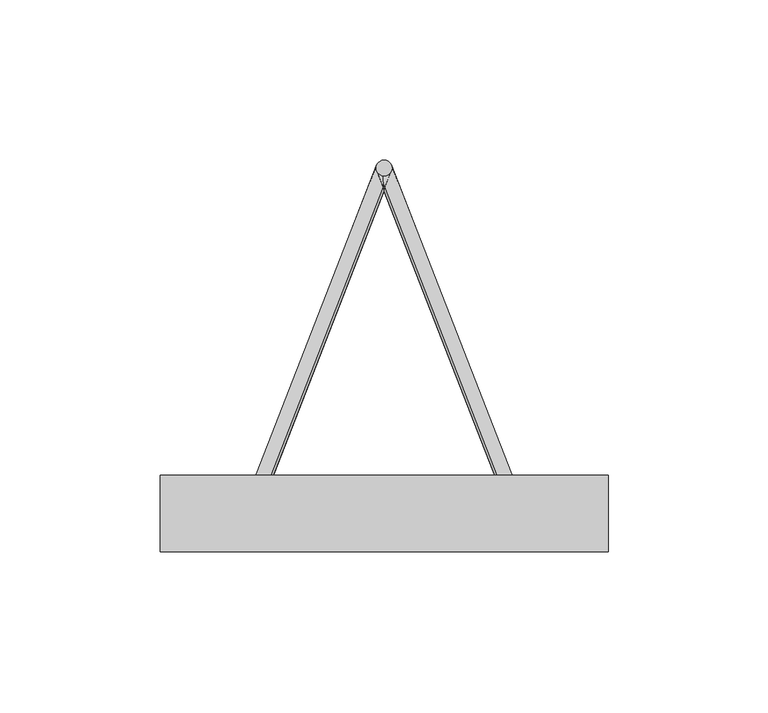
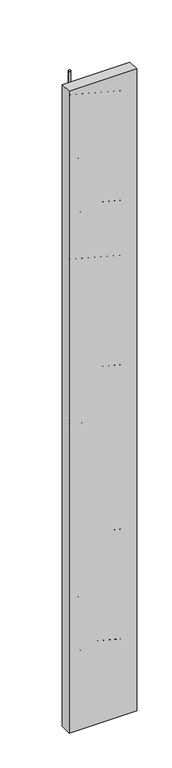
"""IFC4 building model written with IfcOpenShell, lengths in millimetres: proxy geometry, Vigota 1 (Pano 21) (Mf = 156)."""

from ifc_helpers import new_model, si_unit, point, frame, frame_2d, origin, origin_with_axes, origin_2d, place, context, project, spatial, polyline, circle_curve, trimmed, segment, composite_curve, outline, extrude, source, transform, mapped, element, save


def structural_framing_4ac9c4cf(model_context):
    return source(origin(), model_context, "Body", "SweptSolid", [
        extrude(outline(polyline([(-70.0, 12.0), (70.0, 12.0), (70.0, -12.0), (-70.0, -12.0), (-70.0, 12.0)])), origin_with_axes(), (0.0, 0.0, 1.0), 1404.99893),
        extrude(outline(composite_curve([segment(trimmed(circle_curve(frame_2d((42.0, 0.0)), 2.5), [point((44.5, 0.0))], [point((39.5, 0.0))], False, "CARTESIAN"), True, "CONTINUOUS"), segment(trimmed(circle_curve(frame_2d((42.0, 0.0)), 2.5), [point((39.5, 0.0))], [point((44.5, 0.0))], False, "CARTESIAN"), True, "CONTINUOUS")], self_intersect=False)), frame((0.0, 0.0, 28.0), z_axis=(0.0, 0.0, 1.0), x_axis=(1.0, 0.0, 0.0)), (0.0, 0.0, 1.0), 1348.99893),
        extrude(outline(composite_curve([segment(trimmed(circle_curve(frame_2d((0.0, 108.0)), 2.5), [point((2.5, 108.0))], [point((-2.5, 108.0))], False, "CARTESIAN"), True, "CONTINUOUS"), segment(trimmed(circle_curve(frame_2d((0.0, 108.0)), 2.5), [point((-2.5, 108.0))], [point((2.5, 108.0))], False, "CARTESIAN"), True, "CONTINUOUS")], self_intersect=False)), frame((0.0, 0.0, 52.499465), z_axis=(0.0, 0.0, 1.0), x_axis=(1.0, 0.0, 0.0)), (0.0, 0.0, 1.0), 1300.0),
        extrude(outline(composite_curve([segment(trimmed(circle_curve(origin_2d(), 2.5), [point((2.5, 0.0))], [point((-2.5, 0.0))], False, "CARTESIAN"), True, "CONTINUOUS"), segment(trimmed(circle_curve(origin_2d(), 2.5), [point((-2.5, 0.0))], [point((2.5, 0.0))], False, "CARTESIAN"), True, "CONTINUOUS")], self_intersect=False)), frame((42.0, 0.0, 42.499465), z_axis=(-0.3218603428886276, 0.8276408817707567, 0.4598004898837537), x_axis=(0.8192319205108605, -3.936835275445103e-11, 0.5734623443750141)), (0.0, 0.0, 1.0), 130.491379),
        extrude(outline(composite_curve([segment(trimmed(circle_curve(origin_2d(), 2.5), [point((2.5, 0.0))], [point((-2.5, 0.0))], False, "CARTESIAN"), True, "CONTINUOUS"), segment(trimmed(circle_curve(origin_2d(), 2.5), [point((-2.5, 0.0))], [point((2.5, 0.0))], False, "CARTESIAN"), True, "CONTINUOUS")], self_intersect=False)), frame((0.0, 108.0, 102.499465), z_axis=(0.3218603428886276, -0.8276408817707567, 0.4598004898837537), x_axis=(0.8192319205108605, -3.936835275445103e-11, -0.5734623443750141)), (0.0, 0.0, 1.0), 130.491379),
        extrude(outline(composite_curve([segment(trimmed(circle_curve(origin_2d(), 2.5), [point((2.5, 0.0))], [point((-2.5, 0.0))], False, "CARTESIAN"), True, "CONTINUOUS"), segment(trimmed(circle_curve(origin_2d(), 2.5), [point((-2.5, 0.0))], [point((2.5, 0.0))], False, "CARTESIAN"), True, "CONTINUOUS")], self_intersect=False)), frame((42.0, 0.0, 162.499465), z_axis=(-0.3218603428886276, 0.8276408817707567, 0.4598004898837537), x_axis=(0.8192319205108605, -3.936835275445103e-11, 0.5734623443750141)), (0.0, 0.0, 1.0), 130.491379),
        extrude(outline(composite_curve([segment(trimmed(circle_curve(origin_2d(), 2.5), [point((2.5, 0.0))], [point((-2.5, 0.0))], False, "CARTESIAN"), True, "CONTINUOUS"), segment(trimmed(circle_curve(origin_2d(), 2.5), [point((-2.5, 0.0))], [point((2.5, 0.0))], False, "CARTESIAN"), True, "CONTINUOUS")], self_intersect=False)), frame((0.0, 108.0, 222.499465), z_axis=(0.3218603428886276, -0.8276408817707567, 0.4598004898837537), x_axis=(0.8192319205108605, -3.936835275445103e-11, -0.5734623443750141)), (0.0, 0.0, 1.0), 130.491379),
        extrude(outline(composite_curve([segment(trimmed(circle_curve(origin_2d(), 2.5), [point((2.5, 0.0))], [point((-2.5, 0.0))], False, "CARTESIAN"), True, "CONTINUOUS"), segment(trimmed(circle_curve(origin_2d(), 2.5), [point((-2.5, 0.0))], [point((2.5, 0.0))], False, "CARTESIAN"), True, "CONTINUOUS")], self_intersect=False)), frame((42.0, 0.0, 282.499465), z_axis=(-0.3218603428886276, 0.8276408817707567, 0.4598004898837537), x_axis=(0.8192319205108605, -3.936835275445103e-11, 0.5734623443750141)), (0.0, 0.0, 1.0), 130.491379),
        extrude(outline(composite_curve([segment(trimmed(circle_curve(origin_2d(), 2.5), [point((2.5, 0.0))], [point((-2.5, 0.0))], False, "CARTESIAN"), True, "CONTINUOUS"), segment(trimmed(circle_curve(origin_2d(), 2.5), [point((-2.5, 0.0))], [point((2.5, 0.0))], False, "CARTESIAN"), True, "CONTINUOUS")], self_intersect=False)), frame((0.0, 108.0, 342.499465), z_axis=(0.3218603428886276, -0.8276408817707567, 0.4598004898837537), x_axis=(0.8192319205108605, -3.936835275445103e-11, -0.5734623443750141)), (0.0, 0.0, 1.0), 130.491379),
        extrude(outline(composite_curve([segment(trimmed(circle_curve(origin_2d(), 2.5), [point((2.5, 0.0))], [point((-2.5, 0.0))], False, "CARTESIAN"), True, "CONTINUOUS"), segment(trimmed(circle_curve(origin_2d(), 2.5), [point((-2.5, 0.0))], [point((2.5, 0.0))], False, "CARTESIAN"), True, "CONTINUOUS")], self_intersect=False)), frame((42.0, 0.0, 402.499465), z_axis=(-0.3218603428886276, 0.8276408817707567, 0.4598004898837537), x_axis=(0.8192319205108605, -3.936835275445103e-11, 0.5734623443750141)), (0.0, 0.0, 1.0), 130.491379),
        extrude(outline(composite_curve([segment(trimmed(circle_curve(origin_2d(), 2.5), [point((2.5, 0.0))], [point((-2.5, 0.0))], False, "CARTESIAN"), True, "CONTINUOUS"), segment(trimmed(circle_curve(origin_2d(), 2.5), [point((-2.5, 0.0))], [point((2.5, 0.0))], False, "CARTESIAN"), True, "CONTINUOUS")], self_intersect=False)), frame((0.0, 108.0, 462.499465), z_axis=(0.3218603428886276, -0.8276408817707567, 0.4598004898837537), x_axis=(0.8192319205108605, -3.936835275445103e-11, -0.5734623443750141)), (0.0, 0.0, 1.0), 130.491379),
        extrude(outline(composite_curve([segment(trimmed(circle_curve(origin_2d(), 2.5), [point((2.5, 0.0))], [point((-2.5, 0.0))], False, "CARTESIAN"), True, "CONTINUOUS"), segment(trimmed(circle_curve(origin_2d(), 2.5), [point((-2.5, 0.0))], [point((2.5, 0.0))], False, "CARTESIAN"), True, "CONTINUOUS")], self_intersect=False)), frame((42.0, 0.0, 522.499465), z_axis=(-0.3218603428886276, 0.8276408817707567, 0.4598004898837537), x_axis=(0.8192319205108605, -3.936835275445103e-11, 0.5734623443750141)), (0.0, 0.0, 1.0), 130.491379),
        extrude(outline(composite_curve([segment(trimmed(circle_curve(origin_2d(), 2.5), [point((2.5, 0.0))], [point((-2.5, 0.0))], False, "CARTESIAN"), True, "CONTINUOUS"), segment(trimmed(circle_curve(origin_2d(), 2.5), [point((-2.5, 0.0))], [point((2.5, 0.0))], False, "CARTESIAN"), True, "CONTINUOUS")], self_intersect=False)), frame((0.0, 108.0, 582.499465), z_axis=(0.3218603428886276, -0.8276408817707567, 0.4598004898837537), x_axis=(0.8192319205108605, -3.936835275445103e-11, -0.5734623443750141)), (0.0, 0.0, 1.0), 130.491379),
        extrude(outline(composite_curve([segment(trimmed(circle_curve(origin_2d(), 2.5), [point((2.5, 0.0))], [point((-2.5, 0.0))], False, "CARTESIAN"), True, "CONTINUOUS"), segment(trimmed(circle_curve(origin_2d(), 2.5), [point((-2.5, 0.0))], [point((2.5, 0.0))], False, "CARTESIAN"), True, "CONTINUOUS")], self_intersect=False)), frame((42.0, 0.0, 642.499465), z_axis=(-0.3218603428886276, 0.8276408817707567, 0.4598004898837537), x_axis=(0.8192319205108605, -3.936835275445103e-11, 0.5734623443750141)), (0.0, 0.0, 1.0), 130.491379),
        extrude(outline(composite_curve([segment(trimmed(circle_curve(origin_2d(), 2.5), [point((2.5, 0.0))], [point((-2.5, 0.0))], False, "CARTESIAN"), True, "CONTINUOUS"), segment(trimmed(circle_curve(origin_2d(), 2.5), [point((-2.5, 0.0))], [point((2.5, 0.0))], False, "CARTESIAN"), True, "CONTINUOUS")], self_intersect=False)), frame((0.0, 108.0, 702.499465), z_axis=(0.3218603428886276, -0.8276408817707567, 0.4598004898837537), x_axis=(0.8192319205108605, -3.936835275445103e-11, -0.5734623443750141)), (0.0, 0.0, 1.0), 130.491379),
        extrude(outline(composite_curve([segment(trimmed(circle_curve(origin_2d(), 2.5), [point((2.5, 0.0))], [point((-2.5, 0.0))], False, "CARTESIAN"), True, "CONTINUOUS"), segment(trimmed(circle_curve(origin_2d(), 2.5), [point((-2.5, 0.0))], [point((2.5, 0.0))], False, "CARTESIAN"), True, "CONTINUOUS")], self_intersect=False)), frame((42.0, 0.0, 762.499465), z_axis=(-0.3218603428886276, 0.8276408817707567, 0.4598004898837537), x_axis=(0.8192319205108605, -3.936835275445103e-11, 0.5734623443750141)), (0.0, 0.0, 1.0), 130.491379),
        extrude(outline(composite_curve([segment(trimmed(circle_curve(origin_2d(), 2.5), [point((2.5, 0.0))], [point((-2.5, 0.0))], False, "CARTESIAN"), True, "CONTINUOUS"), segment(trimmed(circle_curve(origin_2d(), 2.5), [point((-2.5, 0.0))], [point((2.5, 0.0))], False, "CARTESIAN"), True, "CONTINUOUS")], self_intersect=False)), frame((0.0, 108.0, 822.499465), z_axis=(0.3218603428886276, -0.8276408817707567, 0.4598004898837537), x_axis=(0.8192319205108605, -3.936835275445103e-11, -0.5734623443750141)), (0.0, 0.0, 1.0), 130.491379),
        extrude(outline(composite_curve([segment(trimmed(circle_curve(origin_2d(), 2.5), [point((2.5, 0.0))], [point((-2.5, 0.0))], False, "CARTESIAN"), True, "CONTINUOUS"), segment(trimmed(circle_curve(origin_2d(), 2.5), [point((-2.5, 0.0))], [point((2.5, 0.0))], False, "CARTESIAN"), True, "CONTINUOUS")], self_intersect=False)), frame((42.0, 0.0, 882.499465), z_axis=(-0.3218603428886276, 0.8276408817707567, 0.4598004898837537), x_axis=(0.8192319205108605, -3.936835275445103e-11, 0.5734623443750141)), (0.0, 0.0, 1.0), 130.491379),
        extrude(outline(composite_curve([segment(trimmed(circle_curve(origin_2d(), 2.5), [point((2.5, 0.0))], [point((-2.5, 0.0))], False, "CARTESIAN"), True, "CONTINUOUS"), segment(trimmed(circle_curve(origin_2d(), 2.5), [point((-2.5, 0.0))], [point((2.5, 0.0))], False, "CARTESIAN"), True, "CONTINUOUS")], self_intersect=False)), frame((0.0, 108.0, 942.499465), z_axis=(0.3218603428886276, -0.8276408817707567, 0.4598004898837537), x_axis=(0.8192319205108605, -3.936835275445103e-11, -0.5734623443750141)), (0.0, 0.0, 1.0), 130.491379),
        extrude(outline(composite_curve([segment(trimmed(circle_curve(origin_2d(), 2.5), [point((2.5, 0.0))], [point((-2.5, 0.0))], False, "CARTESIAN"), True, "CONTINUOUS"), segment(trimmed(circle_curve(origin_2d(), 2.5), [point((-2.5, 0.0))], [point((2.5, 0.0))], False, "CARTESIAN"), True, "CONTINUOUS")], self_intersect=False)), frame((42.0, 0.0, 1002.499465), z_axis=(-0.3218603428886276, 0.8276408817707567, 0.4598004898837537), x_axis=(0.8192319205108605, -3.936835275445103e-11, 0.5734623443750141)), (0.0, 0.0, 1.0), 130.491379),
        extrude(outline(composite_curve([segment(trimmed(circle_curve(origin_2d(), 2.5), [point((2.5, 0.0))], [point((-2.5, 0.0))], False, "CARTESIAN"), True, "CONTINUOUS"), segment(trimmed(circle_curve(origin_2d(), 2.5), [point((-2.5, 0.0))], [point((2.5, 0.0))], False, "CARTESIAN"), True, "CONTINUOUS")], self_intersect=False)), frame((0.0, 108.0, 1062.499465), z_axis=(0.3218603428886276, -0.8276408817707567, 0.4598004898837537), x_axis=(0.8192319205108605, -3.936835275445103e-11, -0.5734623443750141)), (0.0, 0.0, 1.0), 130.491379),
        extrude(outline(composite_curve([segment(trimmed(circle_curve(origin_2d(), 2.5), [point((2.5, 0.0))], [point((-2.5, 0.0))], False, "CARTESIAN"), True, "CONTINUOUS"), segment(trimmed(circle_curve(origin_2d(), 2.5), [point((-2.5, 0.0))], [point((2.5, 0.0))], False, "CARTESIAN"), True, "CONTINUOUS")], self_intersect=False)), frame((42.0, 0.0, 1122.499465), z_axis=(-0.3218603428886276, 0.8276408817707567, 0.4598004898837537), x_axis=(0.8192319205108605, -3.936835275445103e-11, 0.5734623443750141)), (0.0, 0.0, 1.0), 130.491379),
        extrude(outline(composite_curve([segment(trimmed(circle_curve(origin_2d(), 2.5), [point((2.5, 0.0))], [point((-2.5, 0.0))], False, "CARTESIAN"), True, "CONTINUOUS"), segment(trimmed(circle_curve(origin_2d(), 2.5), [point((-2.5, 0.0))], [point((2.5, 0.0))], False, "CARTESIAN"), True, "CONTINUOUS")], self_intersect=False)), frame((0.0, 108.0, 1182.499465), z_axis=(0.3218603428886276, -0.8276408817707567, 0.4598004898837537), x_axis=(0.8192319205108605, -3.936835275445103e-11, -0.5734623443750141)), (0.0, 0.0, 1.0), 130.491379),
        extrude(outline(composite_curve([segment(trimmed(circle_curve(origin_2d(), 2.5), [point((2.5, 0.0))], [point((-2.5, 0.0))], False, "CARTESIAN"), True, "CONTINUOUS"), segment(trimmed(circle_curve(origin_2d(), 2.5), [point((-2.5, 0.0))], [point((2.5, 0.0))], False, "CARTESIAN"), True, "CONTINUOUS")], self_intersect=False)), frame((42.0, 0.0, 1242.499465), z_axis=(-0.3218603428886276, 0.8276408817707567, 0.4598004898837537), x_axis=(0.8192319205108605, -3.936835275445103e-11, 0.5734623443750141)), (0.0, 0.0, 1.0), 130.491379),
        extrude(outline(composite_curve([segment(trimmed(circle_curve(origin_2d(), 2.5), [point((2.5, 0.0))], [point((-2.5, 0.0))], False, "CARTESIAN"), True, "CONTINUOUS"), segment(trimmed(circle_curve(origin_2d(), 2.5), [point((-2.5, 0.0))], [point((2.5, 0.0))], False, "CARTESIAN"), True, "CONTINUOUS")], self_intersect=False)), frame((0.0, 108.0, 1302.499465), z_axis=(0.3218603428886276, -0.8276408817707567, 0.4598004898837537), x_axis=(0.8192319205108605, -3.936835275445103e-11, -0.5734623443750141)), (0.0, 0.0, 1.0), 130.491379),
        extrude(outline(composite_curve([segment(trimmed(circle_curve(frame_2d((-42.0, 0.0)), 2.5), [point((-39.5, 0.0))], [point((-44.5, 0.0))], False, "CARTESIAN"), True, "CONTINUOUS"), segment(trimmed(circle_curve(frame_2d((-42.0, 0.0)), 2.5), [point((-44.5, 0.0))], [point((-39.5, 0.0))], False, "CARTESIAN"), True, "CONTINUOUS")], self_intersect=False)), frame((0.0, 0.0, 28.0), z_axis=(0.0, 0.0, 1.0), x_axis=(1.0, 0.0, 0.0)), (0.0, 0.0, 1.0), 1348.99893),
        extrude(outline(composite_curve([segment(trimmed(circle_curve(origin_2d(), 2.5), [point((2.5, 0.0))], [point((-2.5, 0.0))], False, "CARTESIAN"), True, "CONTINUOUS"), segment(trimmed(circle_curve(origin_2d(), 2.5), [point((-2.5, 0.0))], [point((2.5, 0.0))], False, "CARTESIAN"), True, "CONTINUOUS")], self_intersect=False)), frame((-42.0, 0.0, 42.499465), z_axis=(0.3218603428886276, 0.8276408817707567, 0.4598004898837537), x_axis=(0.8192319205108605, 3.936835275445103e-11, -0.5734623443750141)), (0.0, 0.0, 1.0), 130.491379),
        extrude(outline(composite_curve([segment(trimmed(circle_curve(origin_2d(), 2.5), [point((2.5, 0.0))], [point((-2.5, 0.0))], False, "CARTESIAN"), True, "CONTINUOUS"), segment(trimmed(circle_curve(origin_2d(), 2.5), [point((-2.5, 0.0))], [point((2.5, 0.0))], False, "CARTESIAN"), True, "CONTINUOUS")], self_intersect=False)), frame((0.0, 108.0, 102.499465), z_axis=(-0.3218603428886276, -0.8276408817707567, 0.4598004898837537), x_axis=(0.8192319205108605, 3.936835275445103e-11, 0.5734623443750141)), (0.0, 0.0, 1.0), 130.491379),
        extrude(outline(composite_curve([segment(trimmed(circle_curve(origin_2d(), 2.5), [point((2.5, 0.0))], [point((-2.5, 0.0))], False, "CARTESIAN"), True, "CONTINUOUS"), segment(trimmed(circle_curve(origin_2d(), 2.5), [point((-2.5, 0.0))], [point((2.5, 0.0))], False, "CARTESIAN"), True, "CONTINUOUS")], self_intersect=False)), frame((-42.0, 0.0, 162.499465), z_axis=(0.3218603428886276, 0.8276408817707567, 0.4598004898837537), x_axis=(0.8192319205108605, 3.936835275445103e-11, -0.5734623443750141)), (0.0, 0.0, 1.0), 130.491379),
        extrude(outline(composite_curve([segment(trimmed(circle_curve(origin_2d(), 2.5), [point((2.5, 0.0))], [point((-2.5, 0.0))], False, "CARTESIAN"), True, "CONTINUOUS"), segment(trimmed(circle_curve(origin_2d(), 2.5), [point((-2.5, 0.0))], [point((2.5, 0.0))], False, "CARTESIAN"), True, "CONTINUOUS")], self_intersect=False)), frame((0.0, 108.0, 222.499465), z_axis=(-0.3218603428886276, -0.8276408817707567, 0.4598004898837537), x_axis=(0.8192319205108605, 3.936835275445103e-11, 0.5734623443750141)), (0.0, 0.0, 1.0), 130.491379),
        extrude(outline(composite_curve([segment(trimmed(circle_curve(origin_2d(), 2.5), [point((2.5, 0.0))], [point((-2.5, 0.0))], False, "CARTESIAN"), True, "CONTINUOUS"), segment(trimmed(circle_curve(origin_2d(), 2.5), [point((-2.5, 0.0))], [point((2.5, 0.0))], False, "CARTESIAN"), True, "CONTINUOUS")], self_intersect=False)), frame((-42.0, 0.0, 282.499465), z_axis=(0.3218603428886276, 0.8276408817707567, 0.4598004898837537), x_axis=(0.8192319205108605, 3.936835275445103e-11, -0.5734623443750141)), (0.0, 0.0, 1.0), 130.491379),
        extrude(outline(composite_curve([segment(trimmed(circle_curve(origin_2d(), 2.5), [point((2.5, 0.0))], [point((-2.5, 0.0))], False, "CARTESIAN"), True, "CONTINUOUS"), segment(trimmed(circle_curve(origin_2d(), 2.5), [point((-2.5, 0.0))], [point((2.5, 0.0))], False, "CARTESIAN"), True, "CONTINUOUS")], self_intersect=False)), frame((0.0, 108.0, 342.499465), z_axis=(-0.3218603428886276, -0.8276408817707567, 0.4598004898837537), x_axis=(0.8192319205108605, 3.936835275445103e-11, 0.5734623443750141)), (0.0, 0.0, 1.0), 130.491379),
        extrude(outline(composite_curve([segment(trimmed(circle_curve(origin_2d(), 2.5), [point((2.5, 0.0))], [point((-2.5, 0.0))], False, "CARTESIAN"), True, "CONTINUOUS"), segment(trimmed(circle_curve(origin_2d(), 2.5), [point((-2.5, 0.0))], [point((2.5, 0.0))], False, "CARTESIAN"), True, "CONTINUOUS")], self_intersect=False)), frame((-42.0, 0.0, 402.499465), z_axis=(0.3218603428886276, 0.8276408817707567, 0.4598004898837537), x_axis=(0.8192319205108605, 3.936835275445103e-11, -0.5734623443750141)), (0.0, 0.0, 1.0), 130.491379),
        extrude(outline(composite_curve([segment(trimmed(circle_curve(origin_2d(), 2.5), [point((2.5, 0.0))], [point((-2.5, 0.0))], False, "CARTESIAN"), True, "CONTINUOUS"), segment(trimmed(circle_curve(origin_2d(), 2.5), [point((-2.5, 0.0))], [point((2.5, 0.0))], False, "CARTESIAN"), True, "CONTINUOUS")], self_intersect=False)), frame((0.0, 108.0, 462.499465), z_axis=(-0.3218603428886276, -0.8276408817707567, 0.4598004898837537), x_axis=(0.8192319205108605, 3.936835275445103e-11, 0.5734623443750141)), (0.0, 0.0, 1.0), 130.491379),
        extrude(outline(composite_curve([segment(trimmed(circle_curve(origin_2d(), 2.5), [point((2.5, 0.0))], [point((-2.5, 0.0))], False, "CARTESIAN"), True, "CONTINUOUS"), segment(trimmed(circle_curve(origin_2d(), 2.5), [point((-2.5, 0.0))], [point((2.5, 0.0))], False, "CARTESIAN"), True, "CONTINUOUS")], self_intersect=False)), frame((-42.0, 0.0, 522.499465), z_axis=(0.3218603428886276, 0.8276408817707567, 0.4598004898837537), x_axis=(0.8192319205108605, 3.936835275445103e-11, -0.5734623443750141)), (0.0, 0.0, 1.0), 130.491379),
        extrude(outline(composite_curve([segment(trimmed(circle_curve(origin_2d(), 2.5), [point((2.5, 0.0))], [point((-2.5, 0.0))], False, "CARTESIAN"), True, "CONTINUOUS"), segment(trimmed(circle_curve(origin_2d(), 2.5), [point((-2.5, 0.0))], [point((2.5, 0.0))], False, "CARTESIAN"), True, "CONTINUOUS")], self_intersect=False)), frame((0.0, 108.0, 582.499465), z_axis=(-0.3218603428886276, -0.8276408817707567, 0.4598004898837537), x_axis=(0.8192319205108605, 3.936835275445103e-11, 0.5734623443750141)), (0.0, 0.0, 1.0), 130.491379),
        extrude(outline(composite_curve([segment(trimmed(circle_curve(origin_2d(), 2.5), [point((2.5, 0.0))], [point((-2.5, 0.0))], False, "CARTESIAN"), True, "CONTINUOUS"), segment(trimmed(circle_curve(origin_2d(), 2.5), [point((-2.5, 0.0))], [point((2.5, 0.0))], False, "CARTESIAN"), True, "CONTINUOUS")], self_intersect=False)), frame((-42.0, 0.0, 642.499465), z_axis=(0.3218603428886276, 0.8276408817707567, 0.4598004898837537), x_axis=(0.8192319205108605, 3.936835275445103e-11, -0.5734623443750141)), (0.0, 0.0, 1.0), 130.491379),
        extrude(outline(composite_curve([segment(trimmed(circle_curve(origin_2d(), 2.5), [point((2.5, 0.0))], [point((-2.5, 0.0))], False, "CARTESIAN"), True, "CONTINUOUS"), segment(trimmed(circle_curve(origin_2d(), 2.5), [point((-2.5, 0.0))], [point((2.5, 0.0))], False, "CARTESIAN"), True, "CONTINUOUS")], self_intersect=False)), frame((0.0, 108.0, 702.499465), z_axis=(-0.3218603428886276, -0.8276408817707567, 0.4598004898837537), x_axis=(0.8192319205108605, 3.936835275445103e-11, 0.5734623443750141)), (0.0, 0.0, 1.0), 130.491379),
        extrude(outline(composite_curve([segment(trimmed(circle_curve(origin_2d(), 2.5), [point((2.5, 0.0))], [point((-2.5, 0.0))], False, "CARTESIAN"), True, "CONTINUOUS"), segment(trimmed(circle_curve(origin_2d(), 2.5), [point((-2.5, 0.0))], [point((2.5, 0.0))], False, "CARTESIAN"), True, "CONTINUOUS")], self_intersect=False)), frame((-42.0, 0.0, 762.499465), z_axis=(0.3218603428886276, 0.8276408817707567, 0.4598004898837537), x_axis=(0.8192319205108605, 3.936835275445103e-11, -0.5734623443750141)), (0.0, 0.0, 1.0), 130.491379),
        extrude(outline(composite_curve([segment(trimmed(circle_curve(origin_2d(), 2.5), [point((2.5, 0.0))], [point((-2.5, 0.0))], False, "CARTESIAN"), True, "CONTINUOUS"), segment(trimmed(circle_curve(origin_2d(), 2.5), [point((-2.5, 0.0))], [point((2.5, 0.0))], False, "CARTESIAN"), True, "CONTINUOUS")], self_intersect=False)), frame((0.0, 108.0, 822.499465), z_axis=(-0.3218603428886276, -0.8276408817707567, 0.4598004898837537), x_axis=(0.8192319205108605, 3.936835275445103e-11, 0.5734623443750141)), (0.0, 0.0, 1.0), 130.491379),
        extrude(outline(composite_curve([segment(trimmed(circle_curve(origin_2d(), 2.5), [point((2.5, 0.0))], [point((-2.5, 0.0))], False, "CARTESIAN"), True, "CONTINUOUS"), segment(trimmed(circle_curve(origin_2d(), 2.5), [point((-2.5, 0.0))], [point((2.5, 0.0))], False, "CARTESIAN"), True, "CONTINUOUS")], self_intersect=False)), frame((-42.0, 0.0, 882.499465), z_axis=(0.3218603428886276, 0.8276408817707567, 0.4598004898837537), x_axis=(0.8192319205108605, 3.936835275445103e-11, -0.5734623443750141)), (0.0, 0.0, 1.0), 130.491379),
        extrude(outline(composite_curve([segment(trimmed(circle_curve(origin_2d(), 2.5), [point((2.5, 0.0))], [point((-2.5, 0.0))], False, "CARTESIAN"), True, "CONTINUOUS"), segment(trimmed(circle_curve(origin_2d(), 2.5), [point((-2.5, 0.0))], [point((2.5, 0.0))], False, "CARTESIAN"), True, "CONTINUOUS")], self_intersect=False)), frame((0.0, 108.0, 942.499465), z_axis=(-0.3218603428886276, -0.8276408817707567, 0.4598004898837537), x_axis=(0.8192319205108605, 3.936835275445103e-11, 0.5734623443750141)), (0.0, 0.0, 1.0), 130.491379),
        extrude(outline(composite_curve([segment(trimmed(circle_curve(origin_2d(), 2.5), [point((2.5, 0.0))], [point((-2.5, 0.0))], False, "CARTESIAN"), True, "CONTINUOUS"), segment(trimmed(circle_curve(origin_2d(), 2.5), [point((-2.5, 0.0))], [point((2.5, 0.0))], False, "CARTESIAN"), True, "CONTINUOUS")], self_intersect=False)), frame((-42.0, 0.0, 1002.499465), z_axis=(0.3218603428886276, 0.8276408817707567, 0.4598004898837537), x_axis=(0.8192319205108605, 3.936835275445103e-11, -0.5734623443750141)), (0.0, 0.0, 1.0), 130.491379),
        extrude(outline(composite_curve([segment(trimmed(circle_curve(origin_2d(), 2.5), [point((2.5, 0.0))], [point((-2.5, 0.0))], False, "CARTESIAN"), True, "CONTINUOUS"), segment(trimmed(circle_curve(origin_2d(), 2.5), [point((-2.5, 0.0))], [point((2.5, 0.0))], False, "CARTESIAN"), True, "CONTINUOUS")], self_intersect=False)), frame((0.0, 108.0, 1062.499465), z_axis=(-0.3218603428886276, -0.8276408817707567, 0.4598004898837537), x_axis=(0.8192319205108605, 3.936835275445103e-11, 0.5734623443750141)), (0.0, 0.0, 1.0), 130.491379),
        extrude(outline(composite_curve([segment(trimmed(circle_curve(origin_2d(), 2.5), [point((2.5, 0.0))], [point((-2.5, 0.0))], False, "CARTESIAN"), True, "CONTINUOUS"), segment(trimmed(circle_curve(origin_2d(), 2.5), [point((-2.5, 0.0))], [point((2.5, 0.0))], False, "CARTESIAN"), True, "CONTINUOUS")], self_intersect=False)), frame((-42.0, 0.0, 1122.499465), z_axis=(0.3218603428886276, 0.8276408817707567, 0.4598004898837537), x_axis=(0.8192319205108605, 3.936835275445103e-11, -0.5734623443750141)), (0.0, 0.0, 1.0), 130.491379),
        extrude(outline(composite_curve([segment(trimmed(circle_curve(origin_2d(), 2.5), [point((2.5, 0.0))], [point((-2.5, 0.0))], False, "CARTESIAN"), True, "CONTINUOUS"), segment(trimmed(circle_curve(origin_2d(), 2.5), [point((-2.5, 0.0))], [point((2.5, 0.0))], False, "CARTESIAN"), True, "CONTINUOUS")], self_intersect=False)), frame((0.0, 108.0, 1182.499465), z_axis=(-0.3218603428886276, -0.8276408817707567, 0.4598004898837537), x_axis=(0.8192319205108605, 3.936835275445103e-11, 0.5734623443750141)), (0.0, 0.0, 1.0), 130.491379),
        extrude(outline(composite_curve([segment(trimmed(circle_curve(origin_2d(), 2.5), [point((2.5, 0.0))], [point((-2.5, 0.0))], False, "CARTESIAN"), True, "CONTINUOUS"), segment(trimmed(circle_curve(origin_2d(), 2.5), [point((-2.5, 0.0))], [point((2.5, 0.0))], False, "CARTESIAN"), True, "CONTINUOUS")], self_intersect=False)), frame((-42.0, 0.0, 1242.499465), z_axis=(0.3218603428886276, 0.8276408817707567, 0.4598004898837537), x_axis=(0.8192319205108605, 3.936835275445103e-11, -0.5734623443750141)), (0.0, 0.0, 1.0), 130.491379),
        extrude(outline(composite_curve([segment(trimmed(circle_curve(origin_2d(), 2.5), [point((2.5, 0.0))], [point((-2.5, 0.0))], False, "CARTESIAN"), True, "CONTINUOUS"), segment(trimmed(circle_curve(origin_2d(), 2.5), [point((-2.5, 0.0))], [point((2.5, 0.0))], False, "CARTESIAN"), True, "CONTINUOUS")], self_intersect=False)), frame((0.0, 108.0, 1302.499465), z_axis=(-0.3218603428886276, -0.8276408817707567, 0.4598004898837537), x_axis=(0.8192319205108605, 3.936835275445103e-11, 0.5734623443750141)), (0.0, 0.0, 1.0), 130.491379),
    ])


if __name__ == "__main__":
    model = new_model("IFC4")
    model_context = context("Model", 3, world=origin())
    ifc_project = project(units=[si_unit("LENGTHUNIT", "METRE", prefix="MILLI")], contexts=[model_context])
    site = spatial("IfcSite", under=ifc_project)
    building = spatial("IfcBuilding", under=site)
    placement = place(None, origin())
    structural_framing_shape = structural_framing_4ac9c4cf(model_context)
    element("IfcBuildingElementProxy", 1, Name="Vigota 1 (Pano 21) (Mf = 156)", ObjectType="Vigota 1 (Pano 21) (Mf = 156)", at=placement, inside=building, context=model_context, shape_type="MappedRepresentation", body=[
        mapped(structural_framing_shape, transform((0.0, 0.0, 0.0), x_axis=(1.0, 0.0, 0.0), y_axis=(0.0, 1.0, 0.0), z_axis=(0.0, 0.0, 1.0))),
    ])
    save(model, "model.ifc")

# Revit data of these elements
# Element 1 (IfcBuildingElementProxy, "Vigota 1 (Pano 21) (Mf = 156)")
#   Materials on its faces: "Aço", "Concreto armado"
# Materials
#   "Aço": class "Metal", colour RGB 120 120 120, transparency 0, Description = "Aço estrutural A36 grau, ASTM B, acabamento laminado", Cost = 0
#   "Concreto armado": class "Não atribuído", colour RGB 168 169 158, transparency 0
